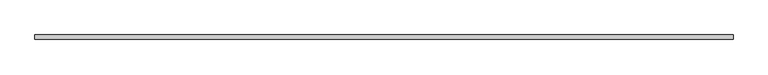
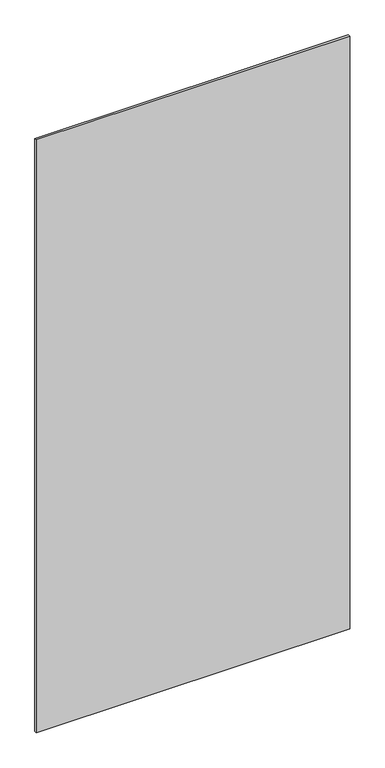
"""IFC4 building model written with IfcOpenShell, lengths in millimetres: proxy geometry, Panel:Panel:300402:Panel:300402 : Panel:Panel:300402:300124:Panel:300402:Panel:300402 : Panel:Panel:300402:300124 : Panel:Panel:300402:Panel:300402 : Panel:Panel:300402:300124:1 : Panel:Panel:300402:Panel:300402 : Panel:Panel:300402:300124:Panel:300402:Panel:300402 : Panel:Panel:300402:300124 : Panel:Panel:300402:Panel:300402 : Panel:Panel:300402:300124:300083."""

from ifc_helpers import new_model, si_unit, frame, origin, place, context, project, spatial, polyline, outline, extrude, source, transform, mapped, element, save


def generic_models_56271434(model_context):
    return source(origin(), model_context, "Body", "SweptSolid", [
        extrude(outline(polyline([(593738.0867239, -579076.8913841), (594957.2867239, -579076.8913841), (594957.2867239, -579084.8288841), (593738.0867239, -579084.8288841), (593738.0867239, -579076.8913841)])), frame((0.0, 0.0, 25.4), z_axis=(0.0, 0.0, 1.0), x_axis=(1.0, 0.0, 0.0)), (0.0, 0.0, 1.0), 2438.4),
    ])


if __name__ == "__main__":
    model = new_model("IFC4")
    model_context = context("Model", 3, world=origin())
    ifc_project = project(units=[si_unit("LENGTHUNIT", "METRE", prefix="MILLI")], contexts=[model_context])
    site = spatial("IfcSite", under=ifc_project)
    building = spatial("IfcBuilding", under=site)
    placement = place(None, origin())
    generic_models_shape = generic_models_56271434(model_context)
    element("IfcBuildingElementProxy", 1, Name="Panel:Panel:300402:Panel:300402 : Panel:Panel:300402:300124:Panel:300402:Panel:300402 : Panel:Panel:300402:300124 : Panel:Panel:300402:Panel:300402 : Panel:Panel:300402:300124:1 : Panel:Panel:300402:Panel:300402 : Panel:Panel:300402:300124:Panel:300402:Panel:300402 : Panel:Panel:300402:300124 : Panel:Panel:300402:Panel:300402 : Panel:Panel:300402:300124:300083", ObjectType="Panel:Panel:300402:Panel:300402 : Panel:Panel:300402:300124:Panel:300402:Panel:300402 : Panel:Panel:300402:300124 : Panel:Panel:300402:Panel:300402 : Panel:Panel:300402:300124:1 : Panel:Panel:300402:Panel:300402 : Panel:Panel:300402:300124:Panel:300402:Panel:300402 : Panel:Panel:300402:300124 : Panel:Panel:300402:Panel:300402 : Panel:Panel:300402:300124:300083", at=placement, inside=building, context=model_context, shape_type="MappedRepresentation", body=[
        mapped(generic_models_shape, transform((0.0, 0.0, 0.0), x_axis=(1.0, 0.0, 0.0), y_axis=(0.0, 1.0, 0.0), z_axis=(0.0, 0.0, 1.0))),
    ])
    save(model, "model.ifc")

# Revit data of these elements
# Type "Panel:Panel:300402:Panel:300402 : Panel:Panel:300402:300124:Panel:300402:Panel:300402 : Panel:Panel:300402:300124 : Panel:Panel:300402:Panel:300402 : Panel:Panel:300402:300124:1 : Panel:Panel:300402:Panel:300402 : Panel:Panel:300402:300124:Panel:300402:Panel:300402 : Panel:Panel:300402:300124 : Panel:Panel:300402:Panel:300402 : Panel:Panel:300402:300124:300083"
#   NameOverride = "Panel:Panel:300402:Panel:300402 : Panel:Panel:300402:300124:Panel:300402:Panel:300402 : Panel:Panel:300402:300124 : Panel:Panel:300402:Panel:300402 : Panel:Panel:300402:300124:300083"
#   ObjectTypeOverride = "Panel:300402:Panel:300402 : Panel:Panel:300402:300124 : Panel:Panel:300402:Panel:300402 : Panel:Panel:300402:300124"
#   Reference = "Panel"
#   Tag = "300083"
# Element 1 (IfcBuildingElementProxy, "Panel:Panel:300402:Panel:300402 : Panel:Panel:300402:300124:Panel:300402:Panel:300402 : Panel:Panel:300402:300124 : Panel:Panel:300402:Panel:300402 : Panel:Panel:300402:300124:1 : Panel:Panel:300402:Panel:300402 : Panel:Panel:300402:300124:Panel:300402:Panel:300402 : Panel:Panel:300402:300124 : Panel:Panel:300402:Panel:300402 : Panel:Panel:300402:300124:300083")
#   Materials on its faces: "5/16\" PHENOLIC RESIN PANELS (CLASS A FLAME SPREAD) - EXPOSED FASTENERS"
# Materials
#   "5/16\" PHENOLIC RESIN PANELS (CLASS A FLAME SPREAD) - EXPOSED FASTENERS": class "Unassigned", colour RGB 64 64 64, transparency 0, Keynote = "M07420000.01", Cost = 0
